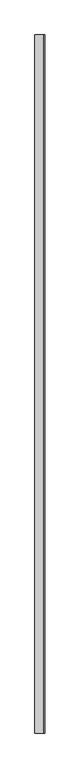
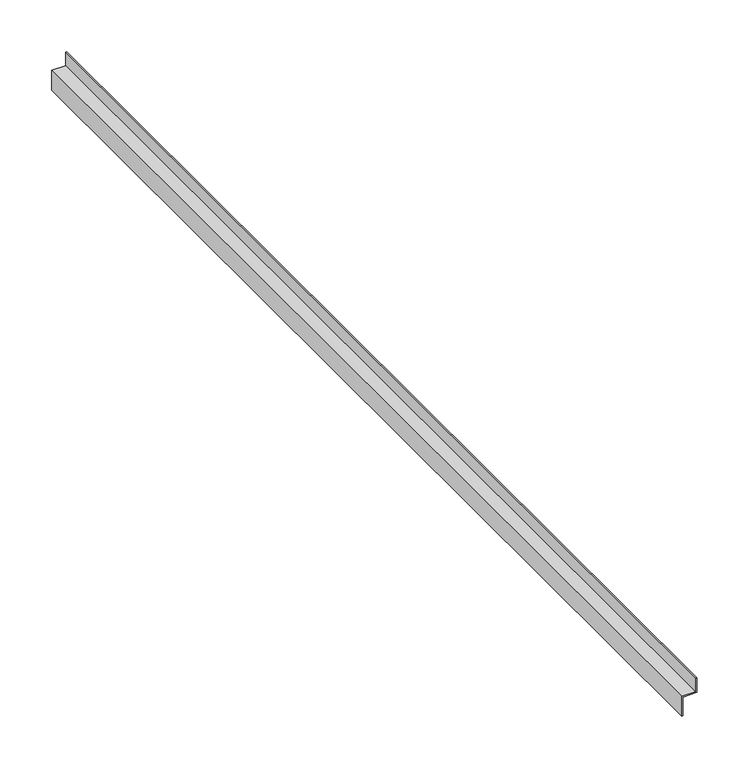
"""IFC4 building model written with IfcOpenShell, lengths in millimetres: proxy geometry, R 092900 - Fry Reglet - Z reveal -  0.049in thick : .625 in Wide Sheating R."""

import ifcopenshell
import ifcopenshell.guid

model = None  # the IFC model being written
_history = None  # IfcOwnerHistory: only IFC2X3 demands one
_inside = {}  # id of a spatial element -> (the spatial element, [elements in it])
_under = {}  # id of a project, library or spatial element -> (it, [spatial elements below it])
_declared = {}  # id of a project -> (the project, [libraries it declares])
_typed = {}  # id of a type object -> (the type object, [elements of that type])
_made_of = {}  # id of a material, layer set ... -> (it, [elements and type objects made of it])


def new_model(schema):
    """Start an empty IFC model of exactly this schema.

    Asked for "IFC4X3", IfcOpenShell would pick the latest addendum, in which some entities
    have other attributes; the version numbers below select the first issue.
    IFC2X3 requires an IfcOwnerHistory on every rooted entity: one is made here for all.
    """
    global model, _history
    if schema == "IFC4X3":
        model = ifcopenshell.file(schema_version=(4, 3, 0, 0))
    else:
        model = ifcopenshell.file(schema=schema)
    _inside.clear()
    _under.clear()
    _declared.clear()
    _typed.clear()
    _made_of.clear()
    _history = None
    if model.schema == "IFC2X3":
        org = make("IfcOrganization", Name="unknown")
        user = make(
            "IfcPersonAndOrganization",
            ThePerson=make("IfcPerson", FamilyName="unknown"),
            TheOrganization=org,
        )
        app = make(
            "IfcApplication",
            ApplicationDeveloper=org,
            Version="unknown",
            ApplicationFullName="unknown",
            ApplicationIdentifier="unknown",
        )
        _history = make(
            "IfcOwnerHistory",
            OwningUser=user,
            OwningApplication=app,
            ChangeAction="ADDED",
            CreationDate=0,
        )
    return model


def make(cls, **values):
    """One entity of the class cls with the attributes given. An attribute that is None is left unset."""
    return model.create_entity(
        cls, **{name: value for name, value in values.items() if value is not None}
    )


def rooted(cls, **values):
    """An entity with a GlobalId (a new one), such as an element, a storey or a relation."""
    return make(cls, GlobalId=ifcopenshell.guid.new(), OwnerHistory=_history, **values)


def si_unit(unit_type, name, prefix=None):
    """IfcSIUnit, for example si_unit("LENGTHUNIT", "METRE", prefix="MILLI")."""
    return make("IfcSIUnit", UnitType=unit_type, Prefix=prefix, Name=name)


def assignment(units):
    """IfcUnitAssignment: the units of a project."""
    return None if units is None else make("IfcUnitAssignment", Units=units)


def point(xyz):
    """IfcCartesianPoint."""
    return None if xyz is None else make("IfcCartesianPoint", Coordinates=xyz)


def direction(xyz):
    """IfcDirection."""
    return None if xyz is None else make("IfcDirection", DirectionRatios=xyz)


def frame(location, z_axis=None, x_axis=None):
    """IfcAxis2Placement3D, a coordinate frame: its origin and axes. An axis left out is left unset."""
    return make(
        "IfcAxis2Placement3D",
        Location=point(location),
        Axis=direction(z_axis),
        RefDirection=direction(x_axis),
    )


def origin():
    """The frame at (0, 0, 0) with its axes left unset."""
    return frame((0.0, 0.0, 0.0))


def place(relative_to, where):
    """IfcLocalPlacement: puts the frame where relative to a parent placement (None: the world)."""
    return make(
        "IfcLocalPlacement", PlacementRelTo=relative_to, RelativePlacement=where
    )


def context(
    kind, dimensions, precision=None, world=None, true_north=None, identifier=None
):
    """IfcGeometricRepresentationContext, for example the 3D "Model" context."""
    return make(
        "IfcGeometricRepresentationContext",
        ContextIdentifier=identifier,
        ContextType=kind,
        CoordinateSpaceDimension=dimensions,
        Precision=precision,
        WorldCoordinateSystem=world,
        TrueNorth=true_north,
    )


def project(units=None, contexts=None):
    """IfcProject with its units and contexts."""
    return rooted(
        "IfcProject",
        Name="project",
        RepresentationContexts=contexts,
        UnitsInContext=assignment(units),
    )


def spatial(cls, under=None, at=None, **own):
    """A site, building, storey or space (cls), placed at a placement, below another one or the project."""
    s = rooted(cls, ObjectPlacement=at, **own)
    if under is not None:
        _under.setdefault(under.id(), (under, []))[1].append(s)
    return s


def polyline(points):
    """IfcPolyline through the points."""
    return make("IfcPolyline", Points=[point(p) for p in points])


def outline(outer, holes=None, kind="AREA"):
    """IfcArbitraryClosedProfileDef: a profile drawn as a closed curve; with holes, ...WithVoids."""
    if holes is None:
        return make("IfcArbitraryClosedProfileDef", ProfileType=kind, OuterCurve=outer)
    return make(
        "IfcArbitraryProfileDefWithVoids",
        ProfileType=kind,
        OuterCurve=outer,
        InnerCurves=holes,
    )


def extrude(swept, where, along, depth):
    """IfcExtrudedAreaSolid: the profile swept, set in the frame where, extruded along a direction by depth."""
    return make(
        "IfcExtrudedAreaSolid",
        SweptArea=swept,
        Position=where,
        ExtrudedDirection=direction(along),
        Depth=depth,
    )


def shape(context_of_items, identifier, shape_type, items):
    """IfcShapeRepresentation: the items that make up one representation, for example the "Body"."""
    return make(
        "IfcShapeRepresentation",
        ContextOfItems=context_of_items,
        RepresentationIdentifier=identifier,
        RepresentationType=shape_type,
        Items=items,
    )


def source(mapping_origin, context_of_items, identifier, shape_type, items):
    """IfcRepresentationMap: a shape defined once, which mapped items show again and again."""
    return make(
        "IfcRepresentationMap",
        MappingOrigin=mapping_origin,
        MappedRepresentation=shape(context_of_items, identifier, shape_type, items),
    )


def transform(
    local_origin,
    x_axis=None,
    y_axis=None,
    z_axis=None,
    scale=None,
    scale2=None,
    scale3=None,
    uniform=True,
):
    """IfcCartesianTransformationOperator3D, or its non-uniform kind. x_axis, y_axis, z_axis: its Axis1, 2, 3."""
    if uniform:
        return make(
            "IfcCartesianTransformationOperator3D",
            Axis1=direction(x_axis),
            Axis2=direction(y_axis),
            LocalOrigin=point(local_origin),
            Scale=scale,
            Axis3=direction(z_axis),
        )
    return make(
        "IfcCartesianTransformationOperator3DnonUniform",
        Axis1=direction(x_axis),
        Axis2=direction(y_axis),
        LocalOrigin=point(local_origin),
        Scale=scale,
        Axis3=direction(z_axis),
        Scale2=scale2,
        Scale3=scale3,
    )


def mapped(mapping_source, mapping_target):
    """IfcMappedItem: shows the shape of a source again, moved by a transform."""
    return make(
        "IfcMappedItem", MappingSource=mapping_source, MappingTarget=mapping_target
    )


def made_of(thing, what):
    """Note that an element or type object is made of a material, layer set ...; save() writes the relation."""
    if what is not None:
        _made_of.setdefault(what.id(), (what, []))[1].append(thing)
    return thing


def element(
    cls,
    number,
    at=None,
    inside=None,
    cuts=None,
    type_object=None,
    material=None,
    context=None,
    identifier="Body",
    shape_type=None,
    held_by="IfcProductDefinitionShape",
    body=None,
    shapes=None,
    **own,
):
    """One element of the class cls, such as IfcWall. Its Tag is "e" and its number.

    at: its placement. inside: the storey or other place that contains it. cuts: it is an
    opening in that element (IfcRelVoidsElement). A single representation is given by context,
    identifier, shape_type and body (its items); several are given by shapes. held_by: the class
    of the entity that holds the representations. save() writes the other relations.
    """
    e = rooted(cls, Tag="e%d" % number, ObjectPlacement=at, **own)
    if body is not None:
        shapes = [shape(context, identifier, shape_type, body)]
    if shapes is not None:
        e.Representation = make(held_by, Representations=shapes)
    if inside is not None:
        _inside.setdefault(inside.id(), (inside, []))[1].append(e)
    if cuts is not None:
        rooted(
            "IfcRelVoidsElement", RelatingBuildingElement=cuts, RelatedOpeningElement=e
        )
    if type_object is not None:
        _typed.setdefault(type_object.id(), (type_object, []))[1].append(e)
    return made_of(e, material)


def aggregate(whole, parts):
    """IfcRelAggregates: a whole, such as a stair, and the parts it consists of."""
    return rooted("IfcRelAggregates", RelatingObject=whole, RelatedObjects=parts)


def save(model, path):
    """Write the relations noted so far, then the file.

    IfcRelAggregates (storeys below a building ...), IfcRelContainedInSpatialStructure (elements
    in a storey), IfcRelDefinesByType, IfcRelAssociatesMaterial and IfcRelDeclares: one each for
    every whole, place, type object, material and project.
    """
    for whole, parts in _under.values():
        aggregate(whole, parts)
    for where, things in _inside.values():
        rooted(
            "IfcRelContainedInSpatialStructure",
            RelatedElements=things,
            RelatingStructure=where,
        )
    for kind, things in _typed.values():
        rooted("IfcRelDefinesByType", RelatedObjects=things, RelatingType=kind)
    for what, things in _made_of.values():
        rooted("IfcRelAssociatesMaterial", RelatedObjects=things, RelatingMaterial=what)
    for by, libraries in _declared.values():
        rooted("IfcRelDeclares", RelatingContext=by, RelatedDefinitions=libraries)
    model.write(path)


def generic_models_397c3c02(model_context):
    return source(origin(), model_context, "Body", "SweptSolid", [
        extrude(outline(polyline([(22.225, 0.0), (39.290625, 0.0), (39.290625, -1.190625), (23.415625, -1.190625), (23.415625, -17.065625), (0.0, -17.065625), (0.0, -15.875), (22.225, -15.875), (22.225, 0.0)])), frame((0.0, -609.6, 0.0), z_axis=(0.0, 1.0, 0.0), x_axis=(0.0, 0.0, 1.0)), (0.0, 0.0, 1.0), 1219.2),
    ])


if __name__ == "__main__":
    model = new_model("IFC4")
    model_context = context("Model", 3, world=origin())
    ifc_project = project(units=[si_unit("LENGTHUNIT", "METRE", prefix="MILLI")], contexts=[model_context])
    site = spatial("IfcSite", under=ifc_project)
    building = spatial("IfcBuilding", under=site)
    placement = place(None, origin())
    generic_models_shape = generic_models_397c3c02(model_context)
    element("IfcBuildingElementProxy", 1, Name="R 092900 - Fry Reglet - Z reveal -  0.049in thick : .625 in Wide Sheating R", ObjectType="R 092900 - Fry Reglet - Z reveal -  0.049in thick : .625 in Wide Sheating R", at=placement, inside=building, context=model_context, shape_type="MappedRepresentation", body=[
        mapped(generic_models_shape, transform((0.0, 0.0, 0.0), x_axis=(1.0, 0.0, 0.0), y_axis=(0.0, 1.0, 0.0), z_axis=(0.0, 0.0, 1.0))),
    ])
    save(model, "model.ifc")

# Revit data of these elements
# Type "R 092900 - Fry Reglet - Z reveal -  0.049in thick : .625 in Wide Sheating R"
#   4' Width = 4' - 0"
#   5/8" Gyp = FRY REGLET REVEAL
# Element 1 (IfcBuildingElementProxy, "R 092900 - Fry Reglet - Z reveal -  0.049in thick : .625 in Wide Sheating R")
#   Materials on its faces: "FRY REGLET REVEAL"
# Materials
#   "FRY REGLET REVEAL": class "Unassigned", colour RGB 246 240 166, transparency 0, Cost = 0
